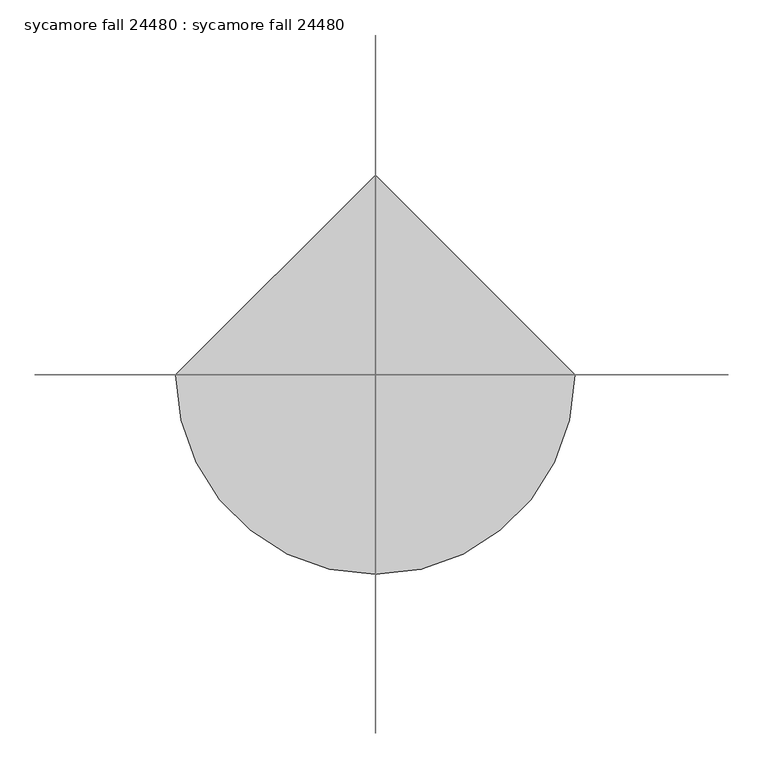
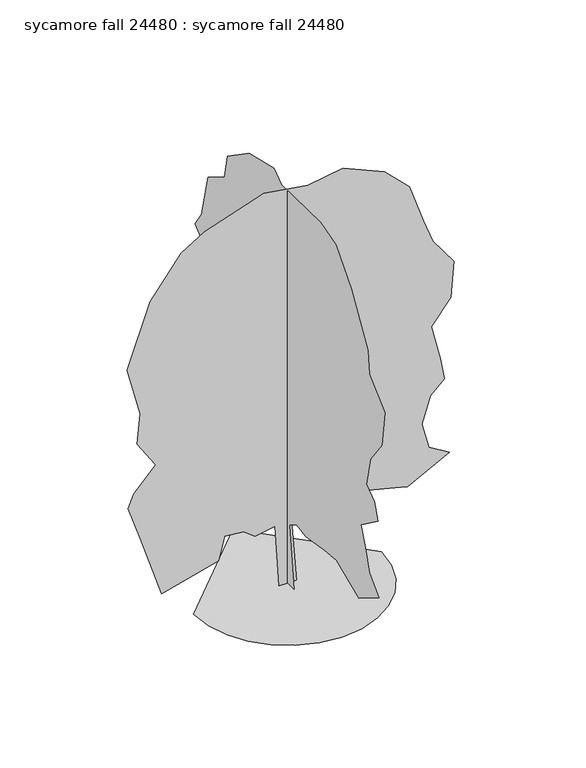
"""IFC4 building model written with IfcOpenShell, lengths in millimetres: proxy geometry, sycamore fall 24480 : sycamore fall 24480."""

import ifcopenshell
import ifcopenshell.guid

model = None  # the IFC model being written
_history = None  # IfcOwnerHistory: only IFC2X3 demands one
_inside = {}  # id of a spatial element -> (the spatial element, [elements in it])
_under = {}  # id of a project, library or spatial element -> (it, [spatial elements below it])
_declared = {}  # id of a project -> (the project, [libraries it declares])
_typed = {}  # id of a type object -> (the type object, [elements of that type])
_made_of = {}  # id of a material, layer set ... -> (it, [elements and type objects made of it])


def new_model(schema):
    """Start an empty IFC model of exactly this schema.

    Asked for "IFC4X3", IfcOpenShell would pick the latest addendum, in which some entities
    have other attributes; the version numbers below select the first issue.
    IFC2X3 requires an IfcOwnerHistory on every rooted entity: one is made here for all.
    """
    global model, _history
    if schema == "IFC4X3":
        model = ifcopenshell.file(schema_version=(4, 3, 0, 0))
    else:
        model = ifcopenshell.file(schema=schema)
    _inside.clear()
    _under.clear()
    _declared.clear()
    _typed.clear()
    _made_of.clear()
    _history = None
    if model.schema == "IFC2X3":
        org = make("IfcOrganization", Name="unknown")
        user = make(
            "IfcPersonAndOrganization",
            ThePerson=make("IfcPerson", FamilyName="unknown"),
            TheOrganization=org,
        )
        app = make(
            "IfcApplication",
            ApplicationDeveloper=org,
            Version="unknown",
            ApplicationFullName="unknown",
            ApplicationIdentifier="unknown",
        )
        _history = make(
            "IfcOwnerHistory",
            OwningUser=user,
            OwningApplication=app,
            ChangeAction="ADDED",
            CreationDate=0,
        )
    return model


def make(cls, **values):
    """One entity of the class cls with the attributes given. An attribute that is None is left unset."""
    return model.create_entity(
        cls, **{name: value for name, value in values.items() if value is not None}
    )


def rooted(cls, **values):
    """An entity with a GlobalId (a new one), such as an element, a storey or a relation."""
    return make(cls, GlobalId=ifcopenshell.guid.new(), OwnerHistory=_history, **values)


def si_unit(unit_type, name, prefix=None):
    """IfcSIUnit, for example si_unit("LENGTHUNIT", "METRE", prefix="MILLI")."""
    return make("IfcSIUnit", UnitType=unit_type, Prefix=prefix, Name=name)


def assignment(units):
    """IfcUnitAssignment: the units of a project."""
    return None if units is None else make("IfcUnitAssignment", Units=units)


def point(xyz):
    """IfcCartesianPoint."""
    return None if xyz is None else make("IfcCartesianPoint", Coordinates=xyz)


def direction(xyz):
    """IfcDirection."""
    return None if xyz is None else make("IfcDirection", DirectionRatios=xyz)


def frame(location, z_axis=None, x_axis=None):
    """IfcAxis2Placement3D, a coordinate frame: its origin and axes. An axis left out is left unset."""
    return make(
        "IfcAxis2Placement3D",
        Location=point(location),
        Axis=direction(z_axis),
        RefDirection=direction(x_axis),
    )


def origin():
    """The frame at (0, 0, 0) with its axes left unset."""
    return frame((0.0, 0.0, 0.0))


def place(relative_to, where):
    """IfcLocalPlacement: puts the frame where relative to a parent placement (None: the world)."""
    return make(
        "IfcLocalPlacement", PlacementRelTo=relative_to, RelativePlacement=where
    )


def context(
    kind, dimensions, precision=None, world=None, true_north=None, identifier=None
):
    """IfcGeometricRepresentationContext, for example the 3D "Model" context."""
    return make(
        "IfcGeometricRepresentationContext",
        ContextIdentifier=identifier,
        ContextType=kind,
        CoordinateSpaceDimension=dimensions,
        Precision=precision,
        WorldCoordinateSystem=world,
        TrueNorth=true_north,
    )


def project(units=None, contexts=None):
    """IfcProject with its units and contexts."""
    return rooted(
        "IfcProject",
        Name="project",
        RepresentationContexts=contexts,
        UnitsInContext=assignment(units),
    )


def spatial(cls, under=None, at=None, **own):
    """A site, building, storey or space (cls), placed at a placement, below another one or the project."""
    s = rooted(cls, ObjectPlacement=at, **own)
    if under is not None:
        _under.setdefault(under.id(), (under, []))[1].append(s)
    return s


def point_list(points):
    """IfcCartesianPointList2D or 3D."""
    cls = (
        "IfcCartesianPointList2D" if len(points[0]) == 2 else "IfcCartesianPointList3D"
    )
    return make(cls, CoordList=points)


def triangles(points, corners, closed=None, point_numbers=None):
    """IfcTriangulatedFaceSet: each triangle names its three corners, points numbered from 1."""
    return make(
        "IfcTriangulatedFaceSet",
        Coordinates=point_list(points),
        Closed=closed,
        CoordIndex=corners,
        PnIndex=point_numbers,
    )


def shape(context_of_items, identifier, shape_type, items):
    """IfcShapeRepresentation: the items that make up one representation, for example the "Body"."""
    return make(
        "IfcShapeRepresentation",
        ContextOfItems=context_of_items,
        RepresentationIdentifier=identifier,
        RepresentationType=shape_type,
        Items=items,
    )


def source(mapping_origin, context_of_items, identifier, shape_type, items):
    """IfcRepresentationMap: a shape defined once, which mapped items show again and again."""
    return make(
        "IfcRepresentationMap",
        MappingOrigin=mapping_origin,
        MappedRepresentation=shape(context_of_items, identifier, shape_type, items),
    )


def transform(
    local_origin,
    x_axis=None,
    y_axis=None,
    z_axis=None,
    scale=None,
    scale2=None,
    scale3=None,
    uniform=True,
):
    """IfcCartesianTransformationOperator3D, or its non-uniform kind. x_axis, y_axis, z_axis: its Axis1, 2, 3."""
    if uniform:
        return make(
            "IfcCartesianTransformationOperator3D",
            Axis1=direction(x_axis),
            Axis2=direction(y_axis),
            LocalOrigin=point(local_origin),
            Scale=scale,
            Axis3=direction(z_axis),
        )
    return make(
        "IfcCartesianTransformationOperator3DnonUniform",
        Axis1=direction(x_axis),
        Axis2=direction(y_axis),
        LocalOrigin=point(local_origin),
        Scale=scale,
        Axis3=direction(z_axis),
        Scale2=scale2,
        Scale3=scale3,
    )


def mapped(mapping_source, mapping_target):
    """IfcMappedItem: shows the shape of a source again, moved by a transform."""
    return make(
        "IfcMappedItem", MappingSource=mapping_source, MappingTarget=mapping_target
    )


def made_of(thing, what):
    """Note that an element or type object is made of a material, layer set ...; save() writes the relation."""
    if what is not None:
        _made_of.setdefault(what.id(), (what, []))[1].append(thing)
    return thing


def element(
    cls,
    number,
    at=None,
    inside=None,
    cuts=None,
    type_object=None,
    material=None,
    context=None,
    identifier="Body",
    shape_type=None,
    held_by="IfcProductDefinitionShape",
    body=None,
    shapes=None,
    **own,
):
    """One element of the class cls, such as IfcWall. Its Tag is "e" and its number.

    at: its placement. inside: the storey or other place that contains it. cuts: it is an
    opening in that element (IfcRelVoidsElement). A single representation is given by context,
    identifier, shape_type and body (its items); several are given by shapes. held_by: the class
    of the entity that holds the representations. save() writes the other relations.
    """
    e = rooted(cls, Tag="e%d" % number, ObjectPlacement=at, **own)
    if body is not None:
        shapes = [shape(context, identifier, shape_type, body)]
    if shapes is not None:
        e.Representation = make(held_by, Representations=shapes)
    if inside is not None:
        _inside.setdefault(inside.id(), (inside, []))[1].append(e)
    if cuts is not None:
        rooted(
            "IfcRelVoidsElement", RelatingBuildingElement=cuts, RelatedOpeningElement=e
        )
    if type_object is not None:
        _typed.setdefault(type_object.id(), (type_object, []))[1].append(e)
    return made_of(e, material)


def aggregate(whole, parts):
    """IfcRelAggregates: a whole, such as a stair, and the parts it consists of."""
    return rooted("IfcRelAggregates", RelatingObject=whole, RelatedObjects=parts)


def save(model, path):
    """Write the relations noted so far, then the file.

    IfcRelAggregates (storeys below a building ...), IfcRelContainedInSpatialStructure (elements
    in a storey), IfcRelDefinesByType, IfcRelAssociatesMaterial and IfcRelDeclares: one each for
    every whole, place, type object, material and project.
    """
    for whole, parts in _under.values():
        aggregate(whole, parts)
    for where, things in _inside.values():
        rooted(
            "IfcRelContainedInSpatialStructure",
            RelatedElements=things,
            RelatingStructure=where,
        )
    for kind, things in _typed.values():
        rooted("IfcRelDefinesByType", RelatedObjects=things, RelatingType=kind)
    for what, things in _made_of.values():
        rooted("IfcRelAssociatesMaterial", RelatedObjects=things, RelatingMaterial=what)
    for by, libraries in _declared.values():
        rooted("IfcRelDeclares", RelatingContext=by, RelatedDefinitions=libraries)
    model.write(path)


def sycamore_fall_24480_sycamore_fall_24480_863b0ace(model_context):
    return source(origin(), model_context, "Body", "Tessellation", [
        triangles([(-350.832074, 1.54e-05, 0.0), (-519.2948653, -0.0002987, 2696.4612831), (-1365.6143188, -0.0002448, 2554.5769203), (-1847.3222706, -0.0002667, 2914.5200661), (-2641.8003754, -0.0002417, 2996.2572281), (-2887.1897575, -0.0001129, 2006.0772606), (-5273.8728561, 6.56e-05, 1384.1309212), (-6175.1399368, -0.000225, 4152.286084), (-6690.1497803, -0.000379, 5632.9271027), (-6446.9198593, -0.0004579, 6205.1631042), (-5531.3774872, -0.0006139, 7177.956633), (-6303.892543, -0.0007221, 8368.8851028), (-6175.1399368, -0.0008812, 9656.4100021), (-6722.3315369, -0.0011105, 11780.8123077), (-5756.700943, -0.001475, 14484.5891327), (-4453.1741135, -0.0017335, 16174.3476196), (-3471.3636932, -0.0018474, 16769.9263824), (-992.8925926, -0.0020555, 17606.8043701), (855.168877, -0.0021033, 17330.758429), (2322.4618732, -0.0021953, 17563.9046631), (4060.6175514, -0.0021804, 16802.108139), (5122.7937057, -0.0021041, 15772.114032), (5702.1926422, -0.001926, 14066.1495575), (6088.4498795, -0.0018163, 13003.948114), (6966.9590469, -0.0017145, 11827.7524658), (6860.9393555, -0.0015239, 10267.9906952), (6024.0607864, -0.0013645, 9237.9704269), (6413.7730453, -0.0011987, 7703.5832703), (6571.2529678, -0.001093, 6759.4920593), (5991.8790298, -0.0010025, 6212.3004593), (5637.8035492, -0.0008488, 5053.5531647), (5937.4468872, -0.0007297, 3944.5144638), (6794.2137772, -0.0007034, 3409.5910103), (5026.248436, -0.000519, 2510.7060516), (4511.2385925, -0.0005118, 2639.4635994), (2708.7041405, -0.0004867, 3090.0846405), (1446.8942413, -0.0004051, 2868.0127304), (1099.3210527, -0.0003972, 2929.1502777), (154.8209641, -0.0004225, 3487.5940979), (137.7651375, -0.0003627, 2991.9900467), (374.3524406, -1.63e-05, 0.0005208), (-4.19e-05, -473.1532413, 0.279514), (8.81e-05, -141.9955024, 2641.8259552), (4.65e-05, -654.9917061, 2992.6504715), (-2.36e-05, -1329.4982094, 2853.8647568), (-0.0001766, -2695.3944878, 3090.3639839), (-0.0002449, -3548.3255653, 3170.8058762), (-0.0004512, -5206.0293228, 2478.7960808), (-0.0005787, -6654.4885849, 3380.0506622), (-0.0004837, -5946.3626221, 4055.9948685), (-0.0004302, -5656.6756531, 4989.4437057), (-0.0003796, -5334.781929, 5826.3222748), (-0.0004627, -6557.9433151, 6727.5893555), (-0.0004219, -6332.6198593, 7435.7153183), (-0.0003424, -5721.0391663, 7854.179892), (-0.0003333, -6010.7261353, 9141.6792114), (-0.0003897, -6847.6297028, 10268.2697479), (-0.0003651, -7072.9275787, 11845.4560364), (-0.0002032, -5962.313974, 12858.9395233), (-0.0001885, -5849.7917725, 13873.2880737), (1.85e-05, -4658.8377228, 15836.7565979), (0.0001585, -3532.2727661, 17124.2814972), (0.0002908, -2408.9233109, 17446.1502228), (0.0005846, 426.8338666, 17381.7867096), (0.0006611, 989.4941082, 17779.9821716), (0.0008252, 2804.4619583, 17349.5793732), (0.0009496, 4340.6016243, 16287.3779297), (0.0009476, 4571.5633987, 15221.4429932), (0.0010368, 5770.0105957, 14484.8681854), (0.0010426, 6252.8386826, 12553.6069977), (0.0010659, 6703.459433, 11845.4560364), (0.0009883, 6168.8153229, 11394.8347046), (0.0009238, 6156.2678329, 9141.6792114), (0.0009203, 6220.656926, 8208.2303741), (0.0008056, 5448.1418701, 7146.0289307), (0.0008789, 6510.3433136, 6180.3977554), (0.0008979, 6703.459433, 5633.2061554), (0.0007283, 6027.5152267, 3219.1165901), (0.0006596, 5350.1995926, 2324.727578), (0.000618, 5264.7798065, 1458.5579189), (0.0004531, 3484.6733459, 1835.0388634), (0.0003699, 2840.9361855, 2156.9174721), (0.0003995, 2647.7947769, 3026.0004707), (0.0002502, 1392.4722725, 2446.6093826), (0.0002126, 1108.5996288, 2659.9106071), (0.0001468, 456.7626357, 2595.6741211), (6.52e-05, 395.9170037, 0.2796182), (-3939.7900429, -8e-07, 0.2427224), (-3835.6501785, -902.7404646, 0.2426104), (-3539.0037506, -1731.7626091, 0.2424986), (-3073.6507599, -2463.3147583, 0.2423909), (-2463.3147583, -3073.6507599, 0.2422916), (-1731.7626091, -3539.0037506, 0.242204), (-902.7404646, -3835.6501785, 0.2421326), (0.0001865, -3939.7900429, 0.2420805), (902.7404646, -3835.6501785, 0.2426061), (1731.7626091, -3539.0037506, 0.2426053), (2463.3147583, -3073.6507599, 0.2426287), (3073.6507599, -2463.3147583, 0.2426749), (3539.0037506, -1731.7626091, 0.2427417), (3835.6501785, -902.7404646, 0.2428276), (3939.7900429, 0.0003444, 0.242378), (-0.0005051, 3939.7900429, 0.2424674)], [[32, 33, 34], [41, 1, 2], [40, 41, 2], [6, 7, 8], [5, 6, 8], [32, 34, 35], [39, 40, 2], [31, 32, 35], [31, 35, 36], [28, 29, 30], [5, 8, 9], [5, 9, 10], [5, 10, 11], [4, 5, 11], [2, 3, 4], [39, 2, 4], [39, 4, 11], [24, 25, 26], [24, 26, 27], [30, 31, 36], [11, 12, 13], [39, 11, 13], [13, 14, 15], [39, 13, 15], [39, 15, 16], [39, 16, 17], [39, 17, 18], [39, 18, 19], [39, 19, 20], [39, 20, 21], [39, 21, 22], [39, 22, 23], [39, 23, 24], [39, 24, 27], [39, 27, 28], [39, 28, 30], [39, 30, 36], [39, 36, 37], [38, 39, 37], [48, 49, 50], [79, 80, 81], [86, 87, 42], [86, 42, 43], [47, 48, 50], [47, 50, 51], [70, 71, 72], [52, 53, 54], [52, 54, 55], [47, 51, 52], [83, 84, 85], [57, 58, 59], [56, 57, 59], [81, 82, 83], [79, 81, 83], [78, 79, 83], [77, 78, 83], [76, 77, 83], [75, 76, 83], [46, 47, 52], [64, 65, 66], [68, 69, 70], [66, 67, 68], [64, 66, 68], [75, 83, 85], [75, 85, 86], [75, 86, 43], [75, 43, 44], [73, 74, 75], [68, 70, 72], [64, 68, 72], [63, 64, 72], [63, 72, 73], [63, 73, 75], [63, 75, 44], [62, 63, 44], [61, 62, 44], [60, 61, 44], [59, 60, 44], [56, 59, 44], [55, 56, 44], [52, 55, 44], [46, 52, 44], [45, 46, 44], [102, 103, 88], [101, 102, 88], [101, 88, 89], [100, 101, 89], [100, 89, 90], [100, 90, 91], [99, 100, 91], [98, 99, 91], [98, 91, 92], [98, 92, 93], [98, 93, 94], [98, 94, 95], [98, 95, 96], [98, 96, 97]], closed=False),
    ])


if __name__ == "__main__":
    model = new_model("IFC4")
    model_context = context("Model", 3, world=origin())
    ifc_project = project(units=[si_unit("LENGTHUNIT", "METRE", prefix="MILLI")], contexts=[model_context])
    site = spatial("IfcSite", under=ifc_project)
    building = spatial("IfcBuilding", under=site)
    placement = place(None, origin())
    sycamore_fall_24480_sycamore_fall_24480_shape = sycamore_fall_24480_sycamore_fall_24480_863b0ace(model_context)
    element("IfcBuildingElementProxy", 1, Name="sycamore fall 24480 : sycamore fall 24480", ObjectType="sycamore fall 24480 : sycamore fall 24480", at=placement, inside=building, context=model_context, shape_type="MappedRepresentation", body=[
        mapped(sycamore_fall_24480_sycamore_fall_24480_shape, transform((0.0, 0.0, 0.0), x_axis=(1.0, 0.0, 0.0), y_axis=(0.0, 1.0, 0.0), z_axis=(0.0, 0.0, 1.0))),
    ])
    save(model, "model.ifc")

# Revit data of these elements
# Type "sycamore fall 24480 : sycamore fall 24480"
#   built-in parameter 1005195 = "RPC-16-G0VS-NDQ0-MUDG-8000-ST1L-LVER-AU"
#   Height = 0
